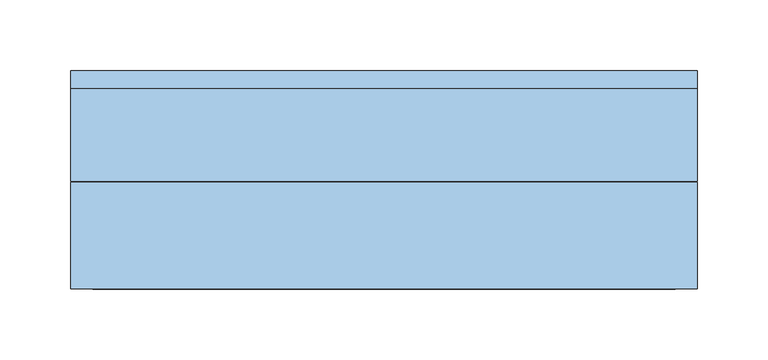
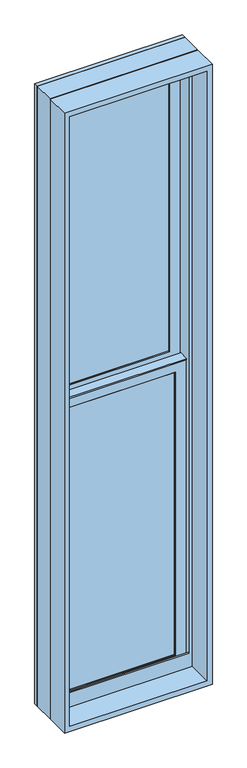
"""IFC4 building model written with IfcOpenShell, lengths in millimetres: window geometry, Window-Double_Hung-Marvin-Essential : ESDH1666."""

from ifc_helpers import new_model, si_unit, frame, origin, place, context, project, spatial, polyline, outline, extrude, faceted_brep, source, transform, mapped, element, save


def window_0775ae5e(model_context):
    return source(origin(), model_context, "Body", "SolidModel", [
        extrude(outline(polyline([(64.5583333, 20.6375), (64.5583333, 15.875), (45.5083333, 15.875), (45.5083333, 20.6375), (64.5583333, 20.6375)])), frame((0.0, 0.0, 527.05), z_axis=(0.0, 0.0, 1.0), x_axis=(1.0, 0.0, 0.0)), (0.0, 0.0, 1.0), 908.05),
        extrude(outline(polyline([(-45.5083333, 20.6375), (-45.5083333, 15.875), (-64.5583333, 15.875), (-64.5583333, 20.6375), (-45.5083333, 20.6375)])), frame((0.0, 0.0, 527.05), z_axis=(0.0, 0.0, 1.0), x_axis=(1.0, 0.0, 0.0)), (0.0, 0.0, 1.0), 908.05),
        extrude(outline(polyline([(165.1, 20.6375), (165.1, 15.875), (-165.1, 15.875), (-165.1, 20.6375), (165.1, 20.6375)])), frame((0.0, 0.0, 971.55), z_axis=(0.0, 0.0, 1.0), x_axis=(1.0, 0.0, 0.0)), (0.0, 0.0, 1.0), 19.05),
        extrude(outline(polyline([(-64.5583333, 46.83125), (-64.5583333, 51.59375), (-45.5083333, 51.59375), (-45.5083333, 46.83125), (-64.5583333, 46.83125)])), frame((0.0, 0.0, 1473.2), z_axis=(0.0, 0.0, 1.0), x_axis=(1.0, 0.0, 0.0)), (0.0, 0.0, 1.0), 908.05),
        extrude(outline(polyline([(45.5083333, 46.83125), (45.5083333, 51.59375), (64.5583333, 51.59375), (64.5583333, 46.83125), (45.5083333, 46.83125)])), frame((0.0, 0.0, 1473.2), z_axis=(0.0, 0.0, 1.0), x_axis=(1.0, 0.0, 0.0)), (0.0, 0.0, 1.0), 908.05),
        extrude(outline(polyline([(-165.1, 46.83125), (-165.1, 51.59375), (165.1, 51.59375), (165.1, 46.83125), (-165.1, 46.83125)])), frame((0.0, 0.0, 1917.7), z_axis=(0.0, 0.0, 1.0), x_axis=(1.0, 0.0, 0.0)), (0.0, 0.0, 1.0), 19.05),
        extrude(outline(polyline([(64.5583333, 20.6375), (45.5083333, 20.6375), (45.5083333, 25.4), (64.5583333, 25.4), (64.5583333, 20.6375)])), frame((0.0, 0.0, 527.05), z_axis=(0.0, 0.0, 1.0), x_axis=(1.0, 0.0, 0.0)), (0.0, 0.0, 1.0), 908.05),
        extrude(outline(polyline([(-45.5083333, 20.6375), (-64.5583333, 20.6375), (-64.5583333, 25.4), (-45.5083333, 25.4), (-45.5083333, 20.6375)])), frame((0.0, 0.0, 527.05), z_axis=(0.0, 0.0, 1.0), x_axis=(1.0, 0.0, 0.0)), (0.0, 0.0, 1.0), 908.05),
        extrude(outline(polyline([(165.1, 20.6375), (-165.1, 20.6375), (-165.1, 25.4), (165.1, 25.4), (165.1, 20.6375)])), frame((0.0, 0.0, 971.55), z_axis=(0.0, 0.0, 1.0), x_axis=(1.0, 0.0, 0.0)), (0.0, 0.0, 1.0), 19.05),
        extrude(outline(polyline([(-64.5583333, 56.35625), (-45.5083333, 56.35625), (-45.5083333, 51.59375), (-64.5583333, 51.59375), (-64.5583333, 56.35625)])), frame((0.0, 0.0, 1473.2), z_axis=(0.0, 0.0, 1.0), x_axis=(1.0, 0.0, 0.0)), (0.0, 0.0, 1.0), 908.05),
        extrude(outline(polyline([(45.5083333, 56.35625), (64.5583333, 56.35625), (64.5583333, 51.59375), (45.5083333, 51.59375), (45.5083333, 56.35625)])), frame((0.0, 0.0, 1473.2), z_axis=(0.0, 0.0, 1.0), x_axis=(1.0, 0.0, 0.0)), (0.0, 0.0, 1.0), 908.05),
        extrude(outline(polyline([(-165.1, 56.35625), (165.1, 56.35625), (165.1, 51.59375), (-165.1, 51.59375), (-165.1, 56.35625)])), frame((0.0, 0.0, 1917.7), z_axis=(0.0, 0.0, 1.0), x_axis=(1.0, 0.0, 0.0)), (0.0, 0.0, 1.0), 19.05),
        faceted_brep([(-192.0875, 5.6780605, 1465.1351748), (-192.0875, 5.6780605, 1460.5), (192.0875, 5.6780605, 1460.5), (192.0875, 5.6780605, 1465.1351748), (-192.0875, 34.8118605, 1465.1351748), (192.0875, 34.8118605, 1465.1351748), (192.0875, 34.8118605, 1460.5), (-192.0875, 34.8118605, 1460.5), (-192.0875, 30.1625, 1460.5), (-192.0875, 30.1625, 500.0625), (-192.0875, 8.9241104, 500.0625), (-192.0875, 8.9241104, 1460.5), (192.0875, 8.9241104, 1460.5), (192.0875, 30.1625, 1460.5), (192.0875, 8.9241104, 500.0625), (192.0875, 30.1625, 500.0625), (-176.2034752, 11.90625, 1446.2034752), (-176.2034752, 30.1625, 1446.2034752), (176.2034752, 30.1625, 1446.2034752), (176.2034752, 11.90625, 1446.2034752), (-159.54375, 10.4662439, 1429.54375), (-159.54375, 11.90625, 1429.54375), (159.54375, 11.90625, 1429.54375), (159.54375, 10.4662439, 1429.54375), (161.0858834, 8.9241104, 1431.0858834), (-161.0858834, 8.9241104, 1431.0858834), (176.2034752, 30.1625, 515.9465248), (176.2034752, 11.90625, 515.9465248), (159.54375, 11.90625, 532.60625), (159.54375, 10.4662439, 532.60625), (161.0858834, 8.9241104, 531.0641166), (-176.2034752, 30.1625, 515.9465248), (-176.2034752, 11.90625, 515.9465248), (-159.54375, 11.90625, 532.60625), (-159.54375, 10.4662439, 532.60625), (-161.0858834, 8.9241104, 531.0641166)], [[[0, 1, 2, 3]], [[4, 5, 6, 7]], [[1, 0, 4, 7, 8, 9, 10, 11]], [[2, 1, 11, 12]], [[7, 6, 13, 8]], [[3, 2, 12, 14, 15, 13, 6, 5]], [[0, 3, 5, 4]], [[16, 17, 18, 19]], [[20, 21, 22, 23]], [[20, 23, 24, 25]], [[19, 18, 26, 27]], [[23, 22, 28, 29]], [[24, 23, 29, 30]], [[27, 26, 31, 32]], [[29, 28, 33, 34]], [[30, 29, 34, 35]], [[15, 14, 10, 9]], [[15, 9, 8, 13], [18, 17, 31, 26]], [[17, 16, 32, 31]], [[16, 19, 27, 32], [22, 21, 33, 28]], [[21, 20, 34, 33]], [[20, 25, 35, 34]], [[10, 14, 12, 11], [25, 24, 30, 35]]]),
        extrude(outline(polyline([(38.5955581, 1446.2125), (33.5778968, 1446.2125), (33.5778968, 1447.8), (39.9405976, 1447.8), (39.9405976, 1446.2125), (61.515625, 1446.2125), (47.6307501, 1442.8975159), (38.5955581, 1442.8975159), (38.5955581, 1446.2125)])), frame((-192.0875, 0.0, 0.0), z_axis=(1.0, 0.0, 0.0), x_axis=(0.0, 1.0, 0.0)), (0.0, 0.0, 1.0), 384.175),
        faceted_brep([(222.25, 0.0, 469.9), (222.25, 0.0, 2438.4), (-222.25, 0.0, 2438.4), (-222.25, 0.0, 469.9), (196.05625, 0.0, 531.01875), (-196.05625, 0.0, 531.01875), (-196.05625, 0.0, 2412.20625), (196.05625, 0.0, 2412.20625), (196.05625, 3.96875, 469.9), (-196.05625, 3.96875, 469.9), (-196.05625, 3.96875, 531.01875), (196.05625, 3.96875, 531.01875), (-222.25, 65.6828125, 469.9), (-196.05625, 65.6828125, 469.9), (196.05625, 65.6828125, 469.9), (222.25, 65.6828125, 469.9), (-222.25, 65.6828125, 2438.4), (222.25, 65.6828125, 2438.4), (196.05625, 65.6828125, 2412.20625), (-196.05625, 65.6828125, 2412.20625)], [[[0, 1, 2, 3], [4, 5, 6, 7]], [[8, 9, 10, 11]], [[5, 4, 11, 10]], [[0, 3, 12, 13, 9, 8, 14, 15]], [[13, 12, 16, 17, 15, 14, 18, 19]], [[13, 19, 6, 5, 10, 9]], [[7, 6, 19, 18]], [[18, 14, 8, 11, 4, 7]], [[1, 0, 15, 17]], [[2, 1, 17, 16]], [[3, 2, 16, 12]]]),
        faceted_brep([(196.05625, 30.1625, 1454.15), (194.46875, 30.1625, 1454.15), (194.46875, 30.1625, 494.2544613), (196.05625, 30.1625, 494.2544613), (-194.46875, 30.1625, 1454.15), (-196.05625, 30.1625, 1454.15), (-196.05625, 30.1625, 494.2544613), (-194.46875, 30.1625, 494.2544613), (194.46875, 63.5, 1454.15), (196.05625, 63.5, 1454.15), (196.05625, 63.5, 487.7743077), (194.46875, 63.5, 487.7743077), (-196.05625, 63.5, 1454.15), (-194.46875, 63.5, 1454.15), (-194.46875, 63.5, 487.7743077), (-196.05625, 63.5, 487.7743077), (207.3108932, 3.96875, 499.3460105), (207.3108932, 3.96875, 469.9), (207.3108932, 65.6828125, 469.9), (207.3108932, 65.6828125, 487.350012), (-207.3108932, 3.96875, 469.9), (-207.3108932, 3.96875, 499.3460105), (-207.3108932, 65.6828125, 487.350012), (-207.3108932, 65.6828125, 469.9), (207.3108932, 78.58125, 484.8428097), (-207.3108932, 78.58125, 484.8428097), (-205.2971252, 68.2348864, 486.8539391), (-187.33135, 68.2348864, 486.8539391), (-187.33135, 65.6828125, 487.350012), (187.33135, 65.6828125, 487.350012), (187.33135, 68.2348864, 486.8539391), (205.2971252, 68.2348864, 486.8539391), (-222.25, 65.6828125, 469.9), (-222.25, 78.5948249, 469.9), (222.25, 78.5948249, 469.9), (222.25, 65.6828125, 469.9), (-222.25, 78.58125, 2438.4), (222.25, 78.58125, 2438.4), (207.3108932, 78.58125, 2423.4608932), (-207.3108932, 78.58125, 2423.4608932), (-222.25, 65.6828125, 2438.4), (-205.2971252, 68.2348864, 2421.4471252), (205.2971252, 68.2348864, 2421.4471252), (187.33135, 68.2348864, 2403.48135), (-187.33135, 68.2348864, 2403.48135), (-187.33135, 65.6828125, 2403.48135), (187.33135, 65.6828125, 2403.48135), (222.25, 65.6828125, 2438.4)], [[[0, 1, 2, 3]], [[4, 5, 6, 7]], [[8, 9, 10, 11]], [[12, 13, 14, 15]], [[1, 8, 11, 2]], [[9, 0, 3, 10]], [[1, 0, 9, 8]], [[5, 4, 13, 12]], [[5, 12, 15, 6]], [[13, 4, 7, 14]], [[16, 17, 18, 19]], [[20, 21, 22, 23]], [[24, 25, 26, 27, 28, 22, 21, 16, 19, 29, 30, 31], [3, 2, 11, 10], [7, 6, 15, 14]], [[17, 16, 21, 20]], [[17, 20, 23, 32, 33, 34, 35, 18]], [[34, 33, 36, 37], [25, 24, 38, 39]], [[33, 32, 40, 36]], [[39, 41, 26, 25]], [[41, 42, 31, 30, 43, 44, 27, 26]], [[44, 45, 28, 27]], [[40, 32, 23, 22, 28, 45, 46, 29, 19, 18, 35, 47]], [[36, 40, 47, 37]], [[39, 38, 42, 41]], [[44, 43, 46, 45]], [[34, 37, 47, 35]], [[42, 38, 24, 31]], [[46, 43, 30, 29]]]),
        extrude(outline(polyline([(172.24375, 11.90625), (-172.24375, 11.90625), (-172.24375, 15.08125), (172.24375, 15.08125), (172.24375, 11.90625)])), frame((0.0, 0.0, 519.90625), z_axis=(0.0, 0.0, 1.0), x_axis=(1.0, 0.0, 0.0)), (0.0, 0.0, 1.0), 922.3375),
        extrude(outline(polyline([(172.24375, 42.8625), (-172.24375, 42.8625), (-172.24375, 46.0375), (172.24375, 46.0375), (172.24375, 42.8625)])), frame((0.0, 0.0, 1466.05625), z_axis=(0.0, 0.0, 1.0), x_axis=(1.0, 0.0, 0.0)), (0.0, 0.0, 1.0), 922.3375),
        faceted_brep([(-159.54375, 31.194477, 1429.54375), (-161.0858834, 32.7366104, 1431.0858834), (161.0858834, 32.7366104, 1431.0858834), (159.54375, 31.194477, 1429.54375), (-159.54375, 30.1625, 1429.54375), (159.54375, 30.1625, 1429.54375), (-192.0875, 32.7366104, 1462.0875), (-192.0875, 30.1625, 1462.0875), (192.0875, 30.1625, 1462.0875), (192.0875, 32.7366104, 1462.0875), (161.0858834, 32.7366104, 531.0641166), (159.54375, 31.194477, 532.60625), (159.54375, 30.1625, 532.60625), (192.0875, 30.1625, 500.0625), (192.0875, 32.7366104, 500.0625), (-161.0858834, 32.7366104, 531.0641166), (-159.54375, 31.194477, 532.60625), (-159.54375, 30.1625, 532.60625), (-192.0875, 30.1625, 500.0625), (-192.0875, 32.7366104, 500.0625)], [[[0, 1, 2, 3]], [[4, 0, 3, 5]], [[6, 7, 8, 9]], [[3, 2, 10, 11]], [[5, 3, 11, 12]], [[9, 8, 13, 14]], [[11, 10, 15, 16]], [[12, 11, 16, 17]], [[14, 13, 18, 19]], [[9, 14, 19, 6], [1, 15, 10, 2]], [[16, 15, 1, 0]], [[17, 16, 0, 4]], [[7, 18, 13, 8], [5, 12, 17, 4]], [[19, 18, 7, 6]]]),
        faceted_brep([(-176.2034752, 42.8625, 2392.3534752), (-176.2034752, 61.11875, 2392.3534752), (176.2034752, 61.11875, 2392.3534752), (176.2034752, 42.8625, 2392.3534752), (-159.54375, 41.4224939, 2375.69375), (-159.54375, 42.8625, 2375.69375), (159.54375, 42.8625, 2375.69375), (159.54375, 41.4224939, 2375.69375), (-161.0858834, 39.8803604, 2377.2358834), (161.0858834, 39.8803604, 2377.2358834), (-192.0875, 61.11875, 2408.2375), (-192.0875, 39.8803604, 2408.2375), (192.0875, 39.8803604, 2408.2375), (192.0875, 61.11875, 2408.2375), (176.2034752, 61.11875, 1462.0965248), (176.2034752, 42.8625, 1462.0965248), (159.54375, 42.8625, 1478.75625), (159.54375, 41.4224939, 1478.75625), (161.0858834, 39.8803604, 1477.2141166), (192.0875, 39.8803604, 1446.2125), (192.0875, 61.11875, 1446.2125), (-176.2034752, 61.11875, 1462.0965248), (-176.2034752, 42.8625, 1462.0965248), (-159.54375, 42.8625, 1478.75625), (-159.54375, 41.4224939, 1478.75625), (-161.0858834, 39.8803604, 1477.2141166), (-192.0875, 39.8803604, 1446.2125), (-192.0875, 61.11875, 1446.2125)], [[[0, 1, 2, 3]], [[4, 5, 6, 7]], [[8, 4, 7, 9]], [[10, 11, 12, 13]], [[3, 2, 14, 15]], [[7, 6, 16, 17]], [[9, 7, 17, 18]], [[13, 12, 19, 20]], [[15, 14, 21, 22]], [[17, 16, 23, 24]], [[18, 17, 24, 25]], [[20, 19, 26, 27]], [[13, 20, 27, 10], [1, 21, 14, 2]], [[22, 21, 1, 0]], [[3, 15, 22, 0], [5, 23, 16, 6]], [[24, 23, 5, 4]], [[25, 24, 4, 8]], [[11, 26, 19, 12], [9, 18, 25, 8]], [[27, 26, 11, 10]]]),
        faceted_brep([(-192.0875, 61.11875, 1446.2125), (-192.0875, 63.6928604, 1446.2125), (192.0875, 63.6928604, 1446.2125), (192.0875, 61.11875, 1446.2125), (-159.54375, 62.150727, 1478.75625), (-159.54375, 61.11875, 1478.75625), (159.54375, 61.11875, 1478.75625), (159.54375, 62.150727, 1478.75625), (-161.0858834, 63.6928604, 1477.2141166), (161.0858834, 63.6928604, 1477.2141166), (192.0875, 63.6928604, 2408.2375), (192.0875, 61.11875, 2408.2375), (159.54375, 61.11875, 2375.69375), (159.54375, 62.150727, 2375.69375), (161.0858834, 63.6928604, 2377.2358834), (-192.0875, 63.6928604, 2408.2375), (-192.0875, 61.11875, 2408.2375), (-159.54375, 61.11875, 2375.69375), (-159.54375, 62.150727, 2375.69375), (-161.0858834, 63.6928604, 2377.2358834)], [[[0, 1, 2, 3]], [[4, 5, 6, 7]], [[8, 4, 7, 9]], [[3, 2, 10, 11]], [[7, 6, 12, 13]], [[9, 7, 13, 14]], [[11, 10, 15, 16]], [[13, 12, 17, 18]], [[14, 13, 18, 19]], [[16, 15, 1, 0]], [[3, 11, 16, 0], [5, 17, 12, 6]], [[18, 17, 5, 4]], [[19, 18, 4, 8]], [[1, 15, 10, 2], [9, 14, 19, 8]]]),
        extrude(outline(polyline([(172.24375, 26.19375), (-172.24375, 26.19375), (-172.24375, 30.1625), (172.24375, 30.1625), (172.24375, 26.19375)])), frame((0.0, 0.0, 519.90625), z_axis=(0.0, 0.0, 1.0), x_axis=(1.0, 0.0, 0.0)), (0.0, 0.0, 1.0), 922.3375),
        extrude(outline(polyline([(172.24375, 57.15), (-172.24375, 57.15), (-172.24375, 61.11875), (172.24375, 61.11875), (172.24375, 57.15)])), frame((0.0, 0.0, 1466.05625), z_axis=(0.0, 0.0, 1.0), x_axis=(1.0, 0.0, 0.0)), (0.0, 0.0, 1.0), 922.3375),
        extrude(outline(polyline([(2438.4, 222.25), (2438.4, -222.25), (469.9, -222.25), (469.9, 222.25), (2438.4, 222.25)]), holes=[polyline([(2422.525, 206.375), (485.775, 206.375), (485.775, -206.375), (2422.525, -206.375), (2422.525, 206.375)])]), frame((0.0, -76.2, 0.0), z_axis=(0.0, 1.0, 0.0), x_axis=(0.0, 0.0, 1.0)), (0.0, 0.0, 1.0), 75.40625),
    ])


if __name__ == "__main__":
    model = new_model("IFC4")
    model_context = context("Model", 3, world=origin())
    ifc_project = project(units=[si_unit("LENGTHUNIT", "METRE", prefix="MILLI")], contexts=[model_context])
    site = spatial("IfcSite", under=ifc_project)
    building = spatial("IfcBuilding", under=site)
    placement = place(None, origin())
    window_shape = window_0775ae5e(model_context)
    element("IfcWindow", 1, ObjectType="Window-Double_Hung-Marvin-Essential : ESDH1666", at=placement, inside=building, context=model_context, shape_type="MappedRepresentation", body=[
        mapped(window_shape, transform((0.0, 0.0, 0.0), x_axis=(1.0, 0.0, 0.0), y_axis=(0.0, 1.0, 0.0), z_axis=(0.0, 0.0, 1.0))),
    ])
    save(model, "model.ifc")

# Revit data of these elements
# Type "Window-Double_Hung-Marvin-Essential : ESDH1666"
#   Type Mark = "82"
#   Window Type = "Essential Double Hung"
#   Product data url = "https://bimobject.com/marvin-windows-and-doors/product/marvin-dhwau"
#   Product Guid = "c4a96547-874c-4385-91dc-a058adc19d98"
#   Frame = "All Ultrex"
#   Egress Window = "No"
#   URL = "www.marvin.com"
#   Model = "ESDH1666"
#   Manufacturer = "Marvin Windows and Doors"
#   Label Egress = ""
#   Glass Type = "IG Low E II with Argon"
#   Design Pressure = "DP40"
#   Description = "1878 DBHG"
#   Analytic Construction = "<None>"
#   Prairie Corner Width = 0' - 4"
#   Prairie Corner Height = 0' - 4"
#   Egress Width = 1' - 2 9/16"
#   Egress Height = 2' - 10 27/128"
#   Rough Width = 1' - 6"
#   Rough Height = 6' - 6"
#   Nominal Width = 1' - 6"
#   Nominal Height = 6' - 6"
#   Inset to Installation Flange [instance default] = 0' - 1"
#   Height = 6' - 5 1/2"
#   Egress Area = 3.4597 SF
#   Default Head Height = 8' - 0"
#   Width = 1' - 5 1/2"
#   Daylight Area = 6.1613 SF
#   DLO Width = 1' - 0 9/16"
#   DLO Height = 2' - 11 5/16"
#   Muntins Top Sash = yes
#   Lites Wide Top Sash = 3
#   Lites Wide Bottom Sash = 3
#   Lites High Top Sash = 2
#   Lites High Bottom Sash = 2
#   Lite Cut Prairie 9 = no
#   Lite Cut HV Grid = yes
#   Muntins Bottom Sash = yes
#   Label Visibility = no
#   Jamb Extension Visibility = yes
#   Edition number = 1
#   Interior Material = Ultrex-Marvin-Stonewhite
#   Glazing Material = Glass-Marvin-IG Low E II with Argon
#   Cladding Material = Ultrex-Marvin-Pebblegray
#   Wall Closure = (empty or 0)
#   Assembly Code = ""
# Element 1 (IfcWindow, "Window-Double_Hung-Marvin-Essential : ESDH1666")
#   Materials on its faces: "Ultrex-Marvin-Pebblegray", "Ultrex-Marvin-Stonewhite", "Glass-Marvin-IG Low E II with Argon"
# Materials
#   "Ultrex-Marvin-Stonewhite": class "Paint", colour RGB 250 251 245, transparency 0
#   "Glass-Marvin-IG Low E II with Argon": class "Glass", colour RGB 0 128 192, transparency 0.85
#   "Ultrex-Marvin-Pebblegray": class "Paint", colour RGB 189 185 173, transparency 0
